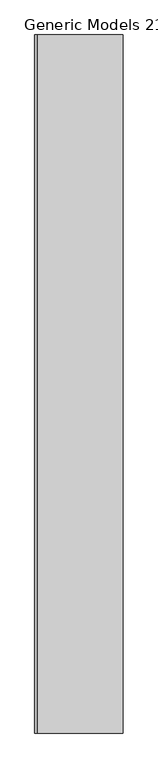
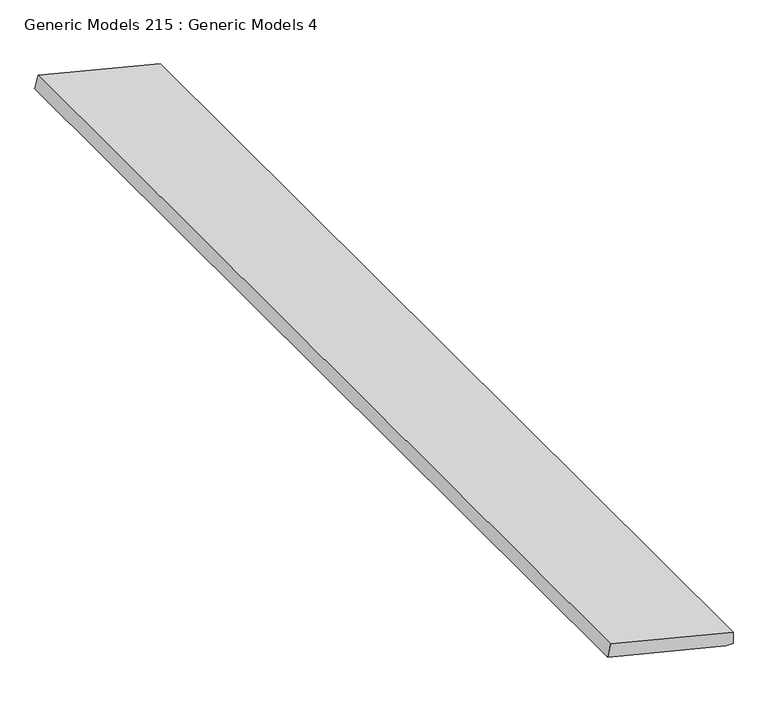
"""IFC4 building model written with IfcOpenShell, lengths in millimetres: proxy geometry, Generic Models 215 : Generic Models 4."""

from ifc_helpers import new_model, si_unit, frame, origin, place, context, project, spatial, polyline, outline, extrude, source, transform, mapped, element, save


def generic_models_215_generic_models_4_044ce0d1(model_context):
    return source(origin(), model_context, "Body", "SweptSolid", [
        extrude(outline(polyline([(129736.1796, 1619.0763704), (130310.5250519, -678.3054374), (130070.2692618, -738.3693849), (129515.8328229, 1479.3763704), (129515.8328229, 1619.0763704), (129736.1796, 1619.0763704)])), frame((0.0, -6864.9230338, 0.0), z_axis=(0.0, 1.0, 0.0), x_axis=(0.0, 0.0, 1.0)), (0.0, 0.0, 1.0), 18643.6),
    ])


if __name__ == "__main__":
    model = new_model("IFC4")
    model_context = context("Model", 3, world=origin())
    ifc_project = project(units=[si_unit("LENGTHUNIT", "METRE", prefix="MILLI")], contexts=[model_context])
    site = spatial("IfcSite", under=ifc_project)
    building = spatial("IfcBuilding", under=site)
    placement = place(None, origin())
    generic_models_215_generic_models_4_shape = generic_models_215_generic_models_4_044ce0d1(model_context)
    element("IfcBuildingElementProxy", 1, Name="Generic Models 215 : Generic Models 4", ObjectType="Generic Models 215 : Generic Models 4", at=placement, inside=building, context=model_context, shape_type="MappedRepresentation", body=[
        mapped(generic_models_215_generic_models_4_shape, transform((0.0, 0.0, 0.0), x_axis=(1.0, 0.0, 0.0), y_axis=(0.0, 1.0, 0.0), z_axis=(0.0, 0.0, 1.0))),
    ])
    save(model, "model.ifc")

# Revit data of these elements
# Element 1 (IfcBuildingElementProxy, "Generic Models 215 : Generic Models 4")
#   Materials on its faces: "_BATT INSUL. (R-FACTOR = R30 MIN) OVER CLASS II VAPOR RETARDER(TOWARD INTERIOR)"
# Materials
#   "_BATT INSUL. (R-FACTOR = R30 MIN) OVER CLASS II VAPOR RETARDER(TOWARD INTERIOR)": class "Generic", colour RGB 200 166 247, transparency 0, Cost = 0
